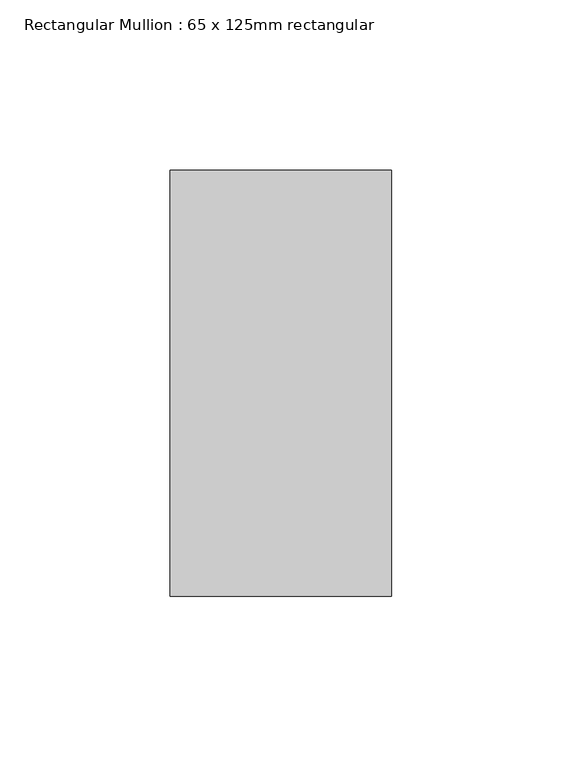
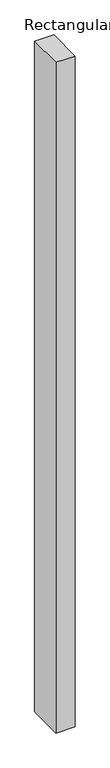
"""IFC4 building model written with IfcOpenShell, lengths in millimetres: member geometry, Rectangular Mullion : 65 x 125mm rectangular."""

from ifc_helpers import new_model, si_unit, frame, origin, place, context, project, spatial, polyline, outline, extrude, source, transform, mapped, element, save


def rectangular_mullion_65_x_125mm_rectangular_8233692a(model_context):
    return source(origin(), model_context, "Body", "SweptSolid", [
        extrude(outline(polyline([(0.0, 62.5), (0.0, -62.5), (-65.0, -62.5), (-65.0, 62.5), (0.0, 62.5)])), frame((0.0, 0.0, -2405.5683179), z_axis=(0.0, 0.0, 1.0), x_axis=(1.0, 0.0, 0.0)), (0.0, 0.0, 1.0), 2405.5683179),
    ])


if __name__ == "__main__":
    model = new_model("IFC4")
    model_context = context("Model", 3, world=origin())
    ifc_project = project(units=[si_unit("LENGTHUNIT", "METRE", prefix="MILLI")], contexts=[model_context])
    site = spatial("IfcSite", under=ifc_project)
    building = spatial("IfcBuilding", under=site)
    placement = place(None, origin())
    rectangular_mullion_65_x_125mm_rectangular_shape = rectangular_mullion_65_x_125mm_rectangular_8233692a(model_context)
    element("IfcMember", 1, ObjectType="Rectangular Mullion : 65 x 125mm rectangular", at=placement, inside=building, context=model_context, shape_type="MappedRepresentation", body=[
        mapped(rectangular_mullion_65_x_125mm_rectangular_shape, transform((0.0, 0.0, 0.0), x_axis=(1.0, 0.0, 0.0), y_axis=(0.0, 1.0, 0.0), z_axis=(0.0, 0.0, 1.0))),
    ])
    save(model, "model.ifc")

# Revit data of these elements
# Type "Rectangular Mullion : 65 x 125mm rectangular"
#   built-in parameter 1007304 = 0.410105 (stored number, unit not read)
#   built-in parameter 1007301 = 0.106627 (stored number, unit not read)
#   built-in parameter 1007300 = 0.106627 (stored number, unit not read)
# Element 1 (IfcMember, "Rectangular Mullion : 65 x 125mm rectangular")
#   Materials on its faces: "Aluminum"
# Materials
#   "Aluminum": class "Metal", colour RGB 244 245 246, transparency 0, Description = "Aluminum 6061", Cost = 0
